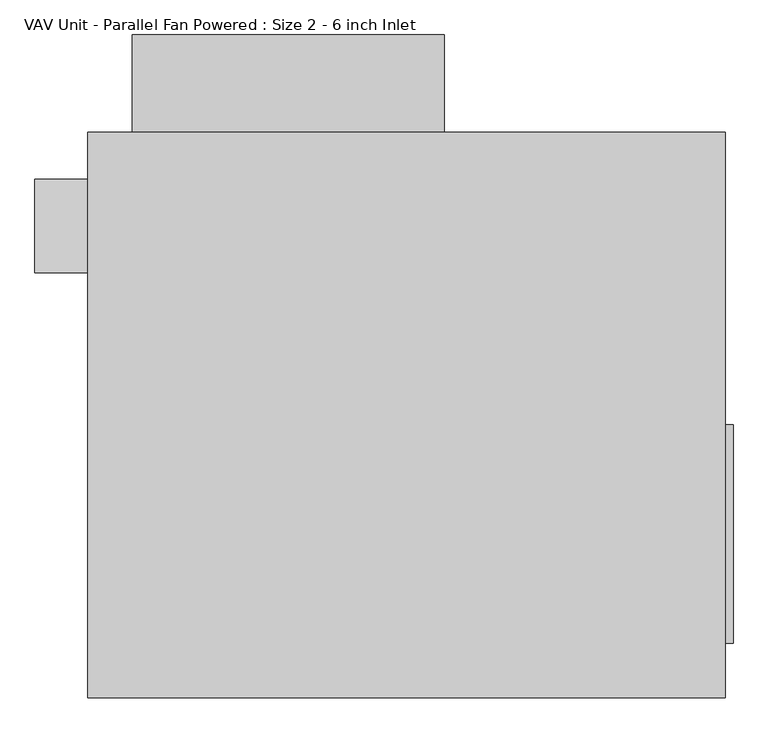
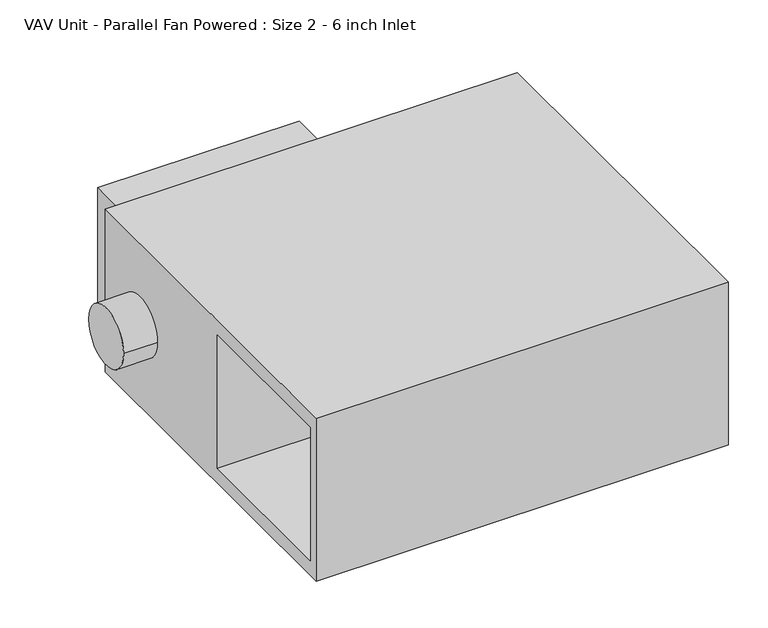
"""IFC4 building model written with IfcOpenShell, lengths in millimetres: proxy geometry, VAV Unit - Parallel Fan Powered : Size 2 - 6 inch Inlet."""

import ifcopenshell
import ifcopenshell.guid

model = None  # the IFC model being written
_history = None  # IfcOwnerHistory: only IFC2X3 demands one
_inside = {}  # id of a spatial element -> (the spatial element, [elements in it])
_under = {}  # id of a project, library or spatial element -> (it, [spatial elements below it])
_declared = {}  # id of a project -> (the project, [libraries it declares])
_typed = {}  # id of a type object -> (the type object, [elements of that type])
_made_of = {}  # id of a material, layer set ... -> (it, [elements and type objects made of it])


def new_model(schema):
    """Start an empty IFC model of exactly this schema.

    Asked for "IFC4X3", IfcOpenShell would pick the latest addendum, in which some entities
    have other attributes; the version numbers below select the first issue.
    IFC2X3 requires an IfcOwnerHistory on every rooted entity: one is made here for all.
    """
    global model, _history
    if schema == "IFC4X3":
        model = ifcopenshell.file(schema_version=(4, 3, 0, 0))
    else:
        model = ifcopenshell.file(schema=schema)
    _inside.clear()
    _under.clear()
    _declared.clear()
    _typed.clear()
    _made_of.clear()
    _history = None
    if model.schema == "IFC2X3":
        org = make("IfcOrganization", Name="unknown")
        user = make(
            "IfcPersonAndOrganization",
            ThePerson=make("IfcPerson", FamilyName="unknown"),
            TheOrganization=org,
        )
        app = make(
            "IfcApplication",
            ApplicationDeveloper=org,
            Version="unknown",
            ApplicationFullName="unknown",
            ApplicationIdentifier="unknown",
        )
        _history = make(
            "IfcOwnerHistory",
            OwningUser=user,
            OwningApplication=app,
            ChangeAction="ADDED",
            CreationDate=0,
        )
    return model


def make(cls, **values):
    """One entity of the class cls with the attributes given. An attribute that is None is left unset."""
    return model.create_entity(
        cls, **{name: value for name, value in values.items() if value is not None}
    )


def rooted(cls, **values):
    """An entity with a GlobalId (a new one), such as an element, a storey or a relation."""
    return make(cls, GlobalId=ifcopenshell.guid.new(), OwnerHistory=_history, **values)


def si_unit(unit_type, name, prefix=None):
    """IfcSIUnit, for example si_unit("LENGTHUNIT", "METRE", prefix="MILLI")."""
    return make("IfcSIUnit", UnitType=unit_type, Prefix=prefix, Name=name)


def assignment(units):
    """IfcUnitAssignment: the units of a project."""
    return None if units is None else make("IfcUnitAssignment", Units=units)


def point(xyz):
    """IfcCartesianPoint."""
    return None if xyz is None else make("IfcCartesianPoint", Coordinates=xyz)


def direction(xyz):
    """IfcDirection."""
    return None if xyz is None else make("IfcDirection", DirectionRatios=xyz)


def frame(location, z_axis=None, x_axis=None):
    """IfcAxis2Placement3D, a coordinate frame: its origin and axes. An axis left out is left unset."""
    return make(
        "IfcAxis2Placement3D",
        Location=point(location),
        Axis=direction(z_axis),
        RefDirection=direction(x_axis),
    )


def frame_2d(location, x_axis=None):
    """IfcAxis2Placement2D, a coordinate frame in the plane: its origin and x axis."""
    return make(
        "IfcAxis2Placement2D", Location=point(location), RefDirection=direction(x_axis)
    )


def origin():
    """The frame at (0, 0, 0) with its axes left unset."""
    return frame((0.0, 0.0, 0.0))


def place(relative_to, where):
    """IfcLocalPlacement: puts the frame where relative to a parent placement (None: the world)."""
    return make(
        "IfcLocalPlacement", PlacementRelTo=relative_to, RelativePlacement=where
    )


def context(
    kind, dimensions, precision=None, world=None, true_north=None, identifier=None
):
    """IfcGeometricRepresentationContext, for example the 3D "Model" context."""
    return make(
        "IfcGeometricRepresentationContext",
        ContextIdentifier=identifier,
        ContextType=kind,
        CoordinateSpaceDimension=dimensions,
        Precision=precision,
        WorldCoordinateSystem=world,
        TrueNorth=true_north,
    )


def project(units=None, contexts=None):
    """IfcProject with its units and contexts."""
    return rooted(
        "IfcProject",
        Name="project",
        RepresentationContexts=contexts,
        UnitsInContext=assignment(units),
    )


def spatial(cls, under=None, at=None, **own):
    """A site, building, storey or space (cls), placed at a placement, below another one or the project."""
    s = rooted(cls, ObjectPlacement=at, **own)
    if under is not None:
        _under.setdefault(under.id(), (under, []))[1].append(s)
    return s


def polyline(points):
    """IfcPolyline through the points."""
    return make("IfcPolyline", Points=[point(p) for p in points])


def circle_curve(where, radius):
    """IfcCircle in the frame where."""
    return make("IfcCircle", Position=where, Radius=radius)


def trimmed(basis, trim1, trim2, sense, master):
    """IfcTrimmedCurve: the piece of a basis curve between two trims."""
    return make(
        "IfcTrimmedCurve",
        BasisCurve=basis,
        Trim1=trim1,
        Trim2=trim2,
        SenseAgreement=sense,
        MasterRepresentation=master,
    )


def segment(curve, same_sense, transition):
    """IfcCompositeCurveSegment."""
    return make(
        "IfcCompositeCurveSegment",
        Transition=transition,
        SameSense=same_sense,
        ParentCurve=curve,
    )


def composite_curve(segments, self_intersect=None):
    """IfcCompositeCurve: segments joined end to end."""
    return make("IfcCompositeCurve", Segments=segments, SelfIntersect=self_intersect)


def outline(outer, holes=None, kind="AREA"):
    """IfcArbitraryClosedProfileDef: a profile drawn as a closed curve; with holes, ...WithVoids."""
    if holes is None:
        return make("IfcArbitraryClosedProfileDef", ProfileType=kind, OuterCurve=outer)
    return make(
        "IfcArbitraryProfileDefWithVoids",
        ProfileType=kind,
        OuterCurve=outer,
        InnerCurves=holes,
    )


def extrude(swept, where, along, depth):
    """IfcExtrudedAreaSolid: the profile swept, set in the frame where, extruded along a direction by depth."""
    return make(
        "IfcExtrudedAreaSolid",
        SweptArea=swept,
        Position=where,
        ExtrudedDirection=direction(along),
        Depth=depth,
    )


def faces_of(points, faces, orient=None, outer=None):
    """IfcFace entities. A face is a list of loops; a loop is a list of indices into points, from 0.

    orient and outer hold one flag for each loop. By default every Orientation is true, the
    first loop of a face is its IfcFaceOuterBound and the others are IfcFaceBound.
    """
    made = []
    for i, loops in enumerate(faces):
        bounds = []
        for j, loop in enumerate(loops):
            is_outer = j == 0 if outer is None else outer[i][j]
            bounds.append(
                make(
                    "IfcFaceOuterBound" if is_outer else "IfcFaceBound",
                    Bound=make("IfcPolyLoop", Polygon=[points[k] for k in loop]),
                    Orientation=True if orient is None else orient[i][j],
                )
            )
        made.append(make("IfcFace", Bounds=bounds))
    return made


def faceted_brep(points, faces, orient=None, outer=None, voids=None):
    """IfcFacetedBrep: a solid bounded by flat faces; with voids (closed shells), ...WithVoids."""
    shared = [point(p) for p in points]
    hull = make("IfcClosedShell", CfsFaces=faces_of(shared, faces, orient, outer))
    if voids is None:
        return make("IfcFacetedBrep", Outer=hull)
    return make(
        "IfcFacetedBrepWithVoids",
        Outer=hull,
        Voids=[
            make(cls, CfsFaces=faces_of(shared, fs, o, b)) for cls, fs, o, b in voids
        ],
    )


def shape(context_of_items, identifier, shape_type, items):
    """IfcShapeRepresentation: the items that make up one representation, for example the "Body"."""
    return make(
        "IfcShapeRepresentation",
        ContextOfItems=context_of_items,
        RepresentationIdentifier=identifier,
        RepresentationType=shape_type,
        Items=items,
    )


def source(mapping_origin, context_of_items, identifier, shape_type, items):
    """IfcRepresentationMap: a shape defined once, which mapped items show again and again."""
    return make(
        "IfcRepresentationMap",
        MappingOrigin=mapping_origin,
        MappedRepresentation=shape(context_of_items, identifier, shape_type, items),
    )


def transform(
    local_origin,
    x_axis=None,
    y_axis=None,
    z_axis=None,
    scale=None,
    scale2=None,
    scale3=None,
    uniform=True,
):
    """IfcCartesianTransformationOperator3D, or its non-uniform kind. x_axis, y_axis, z_axis: its Axis1, 2, 3."""
    if uniform:
        return make(
            "IfcCartesianTransformationOperator3D",
            Axis1=direction(x_axis),
            Axis2=direction(y_axis),
            LocalOrigin=point(local_origin),
            Scale=scale,
            Axis3=direction(z_axis),
        )
    return make(
        "IfcCartesianTransformationOperator3DnonUniform",
        Axis1=direction(x_axis),
        Axis2=direction(y_axis),
        LocalOrigin=point(local_origin),
        Scale=scale,
        Axis3=direction(z_axis),
        Scale2=scale2,
        Scale3=scale3,
    )


def mapped(mapping_source, mapping_target):
    """IfcMappedItem: shows the shape of a source again, moved by a transform."""
    return make(
        "IfcMappedItem", MappingSource=mapping_source, MappingTarget=mapping_target
    )


def made_of(thing, what):
    """Note that an element or type object is made of a material, layer set ...; save() writes the relation."""
    if what is not None:
        _made_of.setdefault(what.id(), (what, []))[1].append(thing)
    return thing


def element(
    cls,
    number,
    at=None,
    inside=None,
    cuts=None,
    type_object=None,
    material=None,
    context=None,
    identifier="Body",
    shape_type=None,
    held_by="IfcProductDefinitionShape",
    body=None,
    shapes=None,
    **own,
):
    """One element of the class cls, such as IfcWall. Its Tag is "e" and its number.

    at: its placement. inside: the storey or other place that contains it. cuts: it is an
    opening in that element (IfcRelVoidsElement). A single representation is given by context,
    identifier, shape_type and body (its items); several are given by shapes. held_by: the class
    of the entity that holds the representations. save() writes the other relations.
    """
    e = rooted(cls, Tag="e%d" % number, ObjectPlacement=at, **own)
    if body is not None:
        shapes = [shape(context, identifier, shape_type, body)]
    if shapes is not None:
        e.Representation = make(held_by, Representations=shapes)
    if inside is not None:
        _inside.setdefault(inside.id(), (inside, []))[1].append(e)
    if cuts is not None:
        rooted(
            "IfcRelVoidsElement", RelatingBuildingElement=cuts, RelatedOpeningElement=e
        )
    if type_object is not None:
        _typed.setdefault(type_object.id(), (type_object, []))[1].append(e)
    return made_of(e, material)


def aggregate(whole, parts):
    """IfcRelAggregates: a whole, such as a stair, and the parts it consists of."""
    return rooted("IfcRelAggregates", RelatingObject=whole, RelatedObjects=parts)


def save(model, path):
    """Write the relations noted so far, then the file.

    IfcRelAggregates (storeys below a building ...), IfcRelContainedInSpatialStructure (elements
    in a storey), IfcRelDefinesByType, IfcRelAssociatesMaterial and IfcRelDeclares: one each for
    every whole, place, type object, material and project.
    """
    for whole, parts in _under.values():
        aggregate(whole, parts)
    for where, things in _inside.values():
        rooted(
            "IfcRelContainedInSpatialStructure",
            RelatedElements=things,
            RelatingStructure=where,
        )
    for kind, things in _typed.values():
        rooted("IfcRelDefinesByType", RelatedObjects=things, RelatingType=kind)
    for what, things in _made_of.values():
        rooted("IfcRelAssociatesMaterial", RelatedObjects=things, RelatingMaterial=what)
    for by, libraries in _declared.values():
        rooted("IfcRelDeclares", RelatingContext=by, RelatedDefinitions=libraries)
    model.write(path)


def vav_unit_parallel_fan_powered_size_2_6_inch_inlet_6222e6d5(model_context):
    return source(origin(), model_context, "Body", "SolidModel", [
        extrude(outline(polyline([(531.8125, -15.875), (531.8125, -371.475), (519.1125, -371.475), (519.1125, -15.875), (531.8125, -15.875)])), frame((0.0, 0.0, -139.7), z_axis=(0.0, 0.0, 1.0), x_axis=(1.0, 0.0, 0.0)), (0.0, 0.0, 1.0), 279.4),
        extrude(outline(polyline([(61.9125, 460.375), (-446.0875, 460.375), (-446.0875, 619.125), (61.9125, 619.125), (61.9125, 460.375)])), frame((0.0, 0.0, -152.4), z_axis=(0.0, 0.0, 1.0), x_axis=(1.0, 0.0, 0.0)), (0.0, 0.0, 1.0), 304.8),
        extrude(outline(composite_curve([segment(trimmed(circle_curve(frame_2d((307.975, 0.0)), 76.2), [point((231.775, 0.0))], [point((384.175, 0.0))], False, "CARTESIAN"), True, "CONTINUOUS"), segment(trimmed(circle_curve(frame_2d((307.975, 0.0)), 76.2), [point((384.175, 0.0))], [point((231.775, 0.0))], False, "CARTESIAN"), True, "CONTINUOUS")], self_intersect=False)), frame((-604.8375, 0.0, 0.0), z_axis=(1.0, 0.0, 0.0), x_axis=(0.0, 1.0, 0.0)), (0.0, 0.0, 1.0), 85.725),
        faceted_brep([(519.1125, 460.375, 217.4875), (-519.1125, 460.375, 217.4875), (-519.1125, -460.375, 217.4875), (519.1125, -460.375, 217.4875), (519.1125, 460.375, -217.4875), (519.1125, -460.375, -217.4875), (-519.1125, -460.375, -217.4875), (-519.1125, 460.375, -217.4875), (-519.1125, -434.975, 177.8), (-519.1125, -434.975, -177.8), (-519.1125, -28.575, -177.8), (-519.1125, -28.575, 177.8), (0.0, -434.975, 177.8), (0.0, -28.575, 177.8), (0.0, -28.575, -177.8), (0.0, -434.975, -177.8)], [[[0, 1, 2, 3]], [[4, 5, 6, 7]], [[1, 0, 4, 7]], [[2, 1, 7, 6], [8, 9, 10, 11]], [[3, 2, 6, 5]], [[0, 3, 5, 4]], [[12, 13, 14, 15]], [[12, 15, 9, 8]], [[15, 14, 10, 9]], [[14, 13, 11, 10]], [[13, 12, 8, 11]]]),
    ])


if __name__ == "__main__":
    model = new_model("IFC4")
    model_context = context("Model", 3, world=origin())
    ifc_project = project(units=[si_unit("LENGTHUNIT", "METRE", prefix="MILLI")], contexts=[model_context])
    site = spatial("IfcSite", under=ifc_project)
    building = spatial("IfcBuilding", under=site)
    placement = place(None, origin())
    vav_unit_parallel_fan_powered_size_2_6_inch_inlet_shape = vav_unit_parallel_fan_powered_size_2_6_inch_inlet_6222e6d5(model_context)
    element("IfcBuildingElementProxy", 1, Name="VAV Unit - Parallel Fan Powered : Size 2 - 6 inch Inlet", ObjectType="VAV Unit - Parallel Fan Powered : Size 2 - 6 inch Inlet", at=placement, inside=building, context=model_context, shape_type="MappedRepresentation", body=[
        mapped(vav_unit_parallel_fan_powered_size_2_6_inch_inlet_shape, transform((0.0, 0.0, 0.0), x_axis=(1.0, 0.0, 0.0), y_axis=(0.0, 1.0, 0.0), z_axis=(0.0, 0.0, 1.0))),
    ])
    save(model, "model.ifc")

# Revit data of these elements
# Type "VAV Unit - Parallel Fan Powered : Size 2 - 6 inch Inlet"
#   Width2 = 1' - 2"
#   Voltage = 120 V
#   UnitWidth = 3' - 4 7/8"
#   UnitHeight = 3' - 0 1/4"
#   UnitDepth = 1' - 5 1/8"
#   SupplyConnectorWidth = 1' - 2"
#   SupplyConnectorVerticalOffset = 0' - 2 1/8"
#   SupplyConnectorLength = 0' - 0 1/2"
#   SupplyConnectorHorizontalOffset = 0' - 3 1/2"
#   SupplyConnectorDepth = 0' - 11"
#   SupplyAirConnectorCenterOffset = 0' - 10 1/2"
#   PrimaryToSupplyRatio [instance default] = 0.2
#   PrimaryAirOffset = 0' - 6"
#   PrimaryAirFlow [instance default] = 100 CFM
#   PrimaryAirConnectorVerticalOffset = 0' - 8 9/16"
#   PrimaryAirConnectorRadius = 0' - 3"
#   PrimaryAirConnectorLength = 0' - 3 3/8"
#   PrimaryAirConnectorDiameter = 0' - 6"
#   PrimaryAirConnectorCenterOffset = 0' - 6"
#   Pressure Drop [instance default] = 0.04 in-wg
#   InducedAirInletWidth = 1' - 4"
#   InducedAirInletDepth = 1' - 2"
#   InducedAirConnectorHorizontalOffset = 0' - 1"
#   InducedAirConnectorCenterOffset = 0' - 9"
#   Height2 = 0' - 11"
#   ElectricalConnectionBoxWidth = 1' - 8"
#   ElectricalConnectionBoxOffset = 0' - 2 7/8"
#   ElectricalConnectionBoxHeight = 0' - 6 1/4"
#   ElectricalConnectionBoxDepth = 1' - 0"
#   SupplyAirFlow [instance default] = 500 CFM
#   Apparent Load = 181 VA
#   SupplyAirConnectorIndex = 2
#   PrimaryAirConnectorIndex = 1
#   Number of Poles = 1
#   InducedAirConnectorIndex = 3
#   VAV Material = none
#   Load Classification = Cooling
#   Assembly Code = ""
